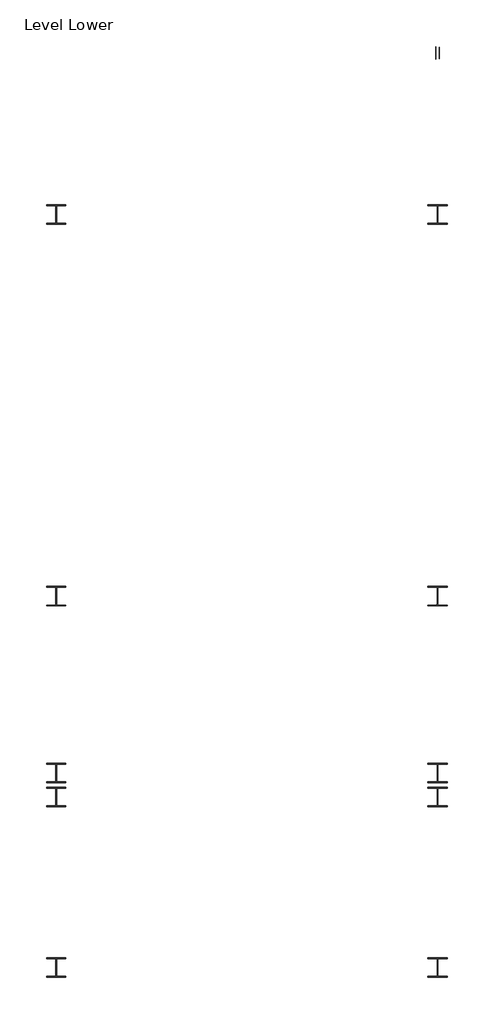
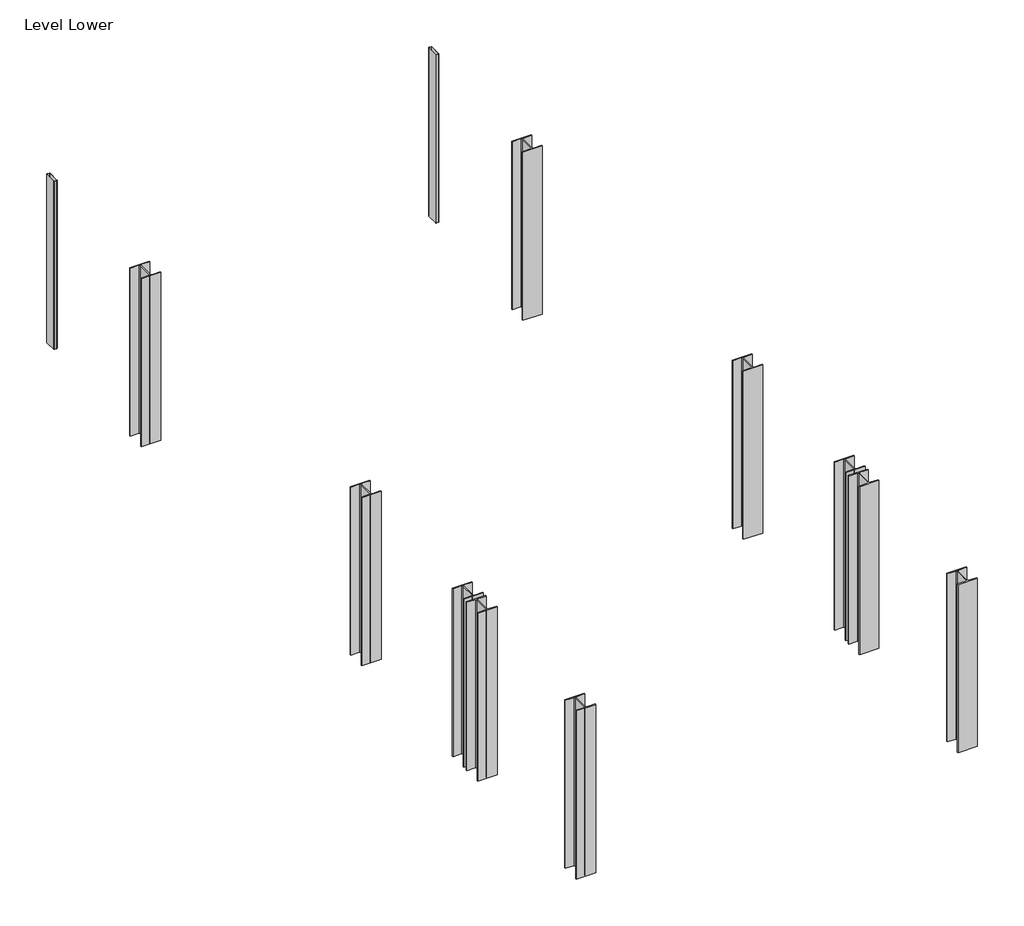
# One storey: 12 columns.
"""IFC4 building model written with IfcOpenShell, lengths in millimetres."""

import ifcopenshell
import ifcopenshell.guid

model = None  # the IFC model being written
_history = None  # IfcOwnerHistory: only IFC2X3 demands one
_inside = {}  # id of a spatial element -> (the spatial element, [elements in it])
_under = {}  # id of a project, library or spatial element -> (it, [spatial elements below it])
_declared = {}  # id of a project -> (the project, [libraries it declares])
_typed = {}  # id of a type object -> (the type object, [elements of that type])
_made_of = {}  # id of a material, layer set ... -> (it, [elements and type objects made of it])


def new_model(schema):
    """Start an empty IFC model of exactly this schema.

    Asked for "IFC4X3", IfcOpenShell would pick the latest addendum, in which some entities
    have other attributes; the version numbers below select the first issue.
    IFC2X3 requires an IfcOwnerHistory on every rooted entity: one is made here for all.
    """
    global model, _history
    if schema == "IFC4X3":
        model = ifcopenshell.file(schema_version=(4, 3, 0, 0))
    else:
        model = ifcopenshell.file(schema=schema)
    _inside.clear()
    _under.clear()
    _declared.clear()
    _typed.clear()
    _made_of.clear()
    _history = None
    if model.schema == "IFC2X3":
        org = make("IfcOrganization", Name="unknown")
        user = make(
            "IfcPersonAndOrganization",
            ThePerson=make("IfcPerson", FamilyName="unknown"),
            TheOrganization=org,
        )
        app = make(
            "IfcApplication",
            ApplicationDeveloper=org,
            Version="unknown",
            ApplicationFullName="unknown",
            ApplicationIdentifier="unknown",
        )
        _history = make(
            "IfcOwnerHistory",
            OwningUser=user,
            OwningApplication=app,
            ChangeAction="ADDED",
            CreationDate=0,
        )
    return model


def make(cls, **values):
    """One entity of the class cls with the attributes given. An attribute that is None is left unset."""
    return model.create_entity(
        cls, **{name: value for name, value in values.items() if value is not None}
    )


def rooted(cls, **values):
    """An entity with a GlobalId (a new one), such as an element, a storey or a relation."""
    return make(cls, GlobalId=ifcopenshell.guid.new(), OwnerHistory=_history, **values)


def si_unit(unit_type, name, prefix=None):
    """IfcSIUnit, for example si_unit("LENGTHUNIT", "METRE", prefix="MILLI")."""
    return make("IfcSIUnit", UnitType=unit_type, Prefix=prefix, Name=name)


def assignment(units):
    """IfcUnitAssignment: the units of a project."""
    return None if units is None else make("IfcUnitAssignment", Units=units)


def point(xyz):
    """IfcCartesianPoint."""
    return None if xyz is None else make("IfcCartesianPoint", Coordinates=xyz)


def direction(xyz):
    """IfcDirection."""
    return None if xyz is None else make("IfcDirection", DirectionRatios=xyz)


def frame(location, z_axis=None, x_axis=None):
    """IfcAxis2Placement3D, a coordinate frame: its origin and axes. An axis left out is left unset."""
    return make(
        "IfcAxis2Placement3D",
        Location=point(location),
        Axis=direction(z_axis),
        RefDirection=direction(x_axis),
    )


def frame_2d(location, x_axis=None):
    """IfcAxis2Placement2D, a coordinate frame in the plane: its origin and x axis."""
    return make(
        "IfcAxis2Placement2D", Location=point(location), RefDirection=direction(x_axis)
    )


def origin():
    """The frame at (0, 0, 0) with its axes left unset."""
    return frame((0.0, 0.0, 0.0))


def place(relative_to, where):
    """IfcLocalPlacement: puts the frame where relative to a parent placement (None: the world)."""
    return make(
        "IfcLocalPlacement", PlacementRelTo=relative_to, RelativePlacement=where
    )


def context(
    kind, dimensions, precision=None, world=None, true_north=None, identifier=None
):
    """IfcGeometricRepresentationContext, for example the 3D "Model" context."""
    return make(
        "IfcGeometricRepresentationContext",
        ContextIdentifier=identifier,
        ContextType=kind,
        CoordinateSpaceDimension=dimensions,
        Precision=precision,
        WorldCoordinateSystem=world,
        TrueNorth=true_north,
    )


def project(units=None, contexts=None):
    """IfcProject with its units and contexts."""
    return rooted(
        "IfcProject",
        Name="project",
        RepresentationContexts=contexts,
        UnitsInContext=assignment(units),
    )


def spatial(cls, under=None, at=None, **own):
    """A site, building, storey or space (cls), placed at a placement, below another one or the project."""
    s = rooted(cls, ObjectPlacement=at, **own)
    if under is not None:
        _under.setdefault(under.id(), (under, []))[1].append(s)
    return s


def polyline(points):
    """IfcPolyline through the points."""
    return make("IfcPolyline", Points=[point(p) for p in points])


def circle_curve(where, radius):
    """IfcCircle in the frame where."""
    return make("IfcCircle", Position=where, Radius=radius)


def trimmed(basis, trim1, trim2, sense, master):
    """IfcTrimmedCurve: the piece of a basis curve between two trims."""
    return make(
        "IfcTrimmedCurve",
        BasisCurve=basis,
        Trim1=trim1,
        Trim2=trim2,
        SenseAgreement=sense,
        MasterRepresentation=master,
    )


def segment(curve, same_sense, transition):
    """IfcCompositeCurveSegment."""
    return make(
        "IfcCompositeCurveSegment",
        Transition=transition,
        SameSense=same_sense,
        ParentCurve=curve,
    )


def composite_curve(segments, self_intersect=None):
    """IfcCompositeCurve: segments joined end to end."""
    return make("IfcCompositeCurve", Segments=segments, SelfIntersect=self_intersect)


def outline(outer, holes=None, kind="AREA"):
    """IfcArbitraryClosedProfileDef: a profile drawn as a closed curve; with holes, ...WithVoids."""
    if holes is None:
        return make("IfcArbitraryClosedProfileDef", ProfileType=kind, OuterCurve=outer)
    return make(
        "IfcArbitraryProfileDefWithVoids",
        ProfileType=kind,
        OuterCurve=outer,
        InnerCurves=holes,
    )


def extrude(swept, where, along, depth):
    """IfcExtrudedAreaSolid: the profile swept, set in the frame where, extruded along a direction by depth."""
    return make(
        "IfcExtrudedAreaSolid",
        SweptArea=swept,
        Position=where,
        ExtrudedDirection=direction(along),
        Depth=depth,
    )


def shape(context_of_items, identifier, shape_type, items):
    """IfcShapeRepresentation: the items that make up one representation, for example the "Body"."""
    return make(
        "IfcShapeRepresentation",
        ContextOfItems=context_of_items,
        RepresentationIdentifier=identifier,
        RepresentationType=shape_type,
        Items=items,
    )


def source(mapping_origin, context_of_items, identifier, shape_type, items):
    """IfcRepresentationMap: a shape defined once, which mapped items show again and again."""
    return make(
        "IfcRepresentationMap",
        MappingOrigin=mapping_origin,
        MappedRepresentation=shape(context_of_items, identifier, shape_type, items),
    )


def transform(
    local_origin,
    x_axis=None,
    y_axis=None,
    z_axis=None,
    scale=None,
    scale2=None,
    scale3=None,
    uniform=True,
):
    """IfcCartesianTransformationOperator3D, or its non-uniform kind. x_axis, y_axis, z_axis: its Axis1, 2, 3."""
    if uniform:
        return make(
            "IfcCartesianTransformationOperator3D",
            Axis1=direction(x_axis),
            Axis2=direction(y_axis),
            LocalOrigin=point(local_origin),
            Scale=scale,
            Axis3=direction(z_axis),
        )
    return make(
        "IfcCartesianTransformationOperator3DnonUniform",
        Axis1=direction(x_axis),
        Axis2=direction(y_axis),
        LocalOrigin=point(local_origin),
        Scale=scale,
        Axis3=direction(z_axis),
        Scale2=scale2,
        Scale3=scale3,
    )


def mapped(mapping_source, mapping_target):
    """IfcMappedItem: shows the shape of a source again, moved by a transform."""
    return make(
        "IfcMappedItem", MappingSource=mapping_source, MappingTarget=mapping_target
    )


def made_of(thing, what):
    """Note that an element or type object is made of a material, layer set ...; save() writes the relation."""
    if what is not None:
        _made_of.setdefault(what.id(), (what, []))[1].append(thing)
    return thing


def element(
    cls,
    number,
    at=None,
    inside=None,
    cuts=None,
    type_object=None,
    material=None,
    context=None,
    identifier="Body",
    shape_type=None,
    held_by="IfcProductDefinitionShape",
    body=None,
    shapes=None,
    **own,
):
    """One element of the class cls, such as IfcWall. Its Tag is "e" and its number.

    at: its placement. inside: the storey or other place that contains it. cuts: it is an
    opening in that element (IfcRelVoidsElement). A single representation is given by context,
    identifier, shape_type and body (its items); several are given by shapes. held_by: the class
    of the entity that holds the representations. save() writes the other relations.
    """
    e = rooted(cls, Tag="e%d" % number, ObjectPlacement=at, **own)
    if body is not None:
        shapes = [shape(context, identifier, shape_type, body)]
    if shapes is not None:
        e.Representation = make(held_by, Representations=shapes)
    if inside is not None:
        _inside.setdefault(inside.id(), (inside, []))[1].append(e)
    if cuts is not None:
        rooted(
            "IfcRelVoidsElement", RelatingBuildingElement=cuts, RelatedOpeningElement=e
        )
    if type_object is not None:
        _typed.setdefault(type_object.id(), (type_object, []))[1].append(e)
    return made_of(e, material)


def aggregate(whole, parts):
    """IfcRelAggregates: a whole, such as a stair, and the parts it consists of."""
    return rooted("IfcRelAggregates", RelatingObject=whole, RelatedObjects=parts)


def save(model, path):
    """Write the relations noted so far, then the file.

    IfcRelAggregates (storeys below a building ...), IfcRelContainedInSpatialStructure (elements
    in a storey), IfcRelDefinesByType, IfcRelAssociatesMaterial and IfcRelDeclares: one each for
    every whole, place, type object, material and project.
    """
    for whole, parts in _under.values():
        aggregate(whole, parts)
    for where, things in _inside.values():
        rooted(
            "IfcRelContainedInSpatialStructure",
            RelatedElements=things,
            RelatingStructure=where,
        )
    for kind, things in _typed.values():
        rooted("IfcRelDefinesByType", RelatedObjects=things, RelatingType=kind)
    for what, things in _made_of.values():
        rooted("IfcRelAssociatesMaterial", RelatedObjects=things, RelatingMaterial=what)
    for by, libraries in _declared.values():
        rooted("IfcRelDeclares", RelatingContext=by, RelatedDefinitions=libraries)
    model.write(path)


def hss_hollow_structural_section_column_hss8x2x3_16_e82f30fd(model_context):
    return source(origin(), model_context, "Body", "SweptSolid", [
        extrude(outline(composite_curve([segment(trimmed(circle_curve(frame_2d((16.5608, 92.7608)), 8.8392), [point((16.5608, 101.6))], [point((25.4, 92.7608))], False, "CARTESIAN"), True, "CONTINUOUS"), segment(polyline([(25.4, 92.7608), (25.4, -92.7608)]), True, "CONTINUOUS"), segment(trimmed(circle_curve(frame_2d((16.5608, -92.7608)), 8.8392), [point((25.4, -92.7608))], [point((16.5608, -101.6))], False, "CARTESIAN"), True, "CONTINUOUS"), segment(polyline([(16.5608, -101.6), (-16.5608, -101.6)]), True, "CONTINUOUS"), segment(trimmed(circle_curve(frame_2d((-16.5608, -92.7608)), 8.8392), [point((-16.5608, -101.6))], [point((-25.4, -92.7608))], False, "CARTESIAN"), True, "CONTINUOUS"), segment(polyline([(-25.4, -92.7608), (-25.4, 92.7608)]), True, "CONTINUOUS"), segment(trimmed(circle_curve(frame_2d((-16.5608, 92.7608)), 8.8392), [point((-25.4, 92.7608))], [point((-16.5608, 101.6))], False, "CARTESIAN"), True, "CONTINUOUS"), segment(polyline([(-16.5608, 101.6), (16.5608, 101.6)]), True, "CONTINUOUS")], self_intersect=False), holes=[composite_curve([segment(polyline([(16.5608, 97.1804), (-16.5608, 97.1804)]), True, "CONTINUOUS"), segment(trimmed(circle_curve(frame_2d((-16.5608, 92.7608)), 4.4196), [point((-16.5608, 97.1804))], [point((-20.9804, 92.7608))], True, "CARTESIAN"), True, "CONTINUOUS"), segment(polyline([(-20.9804, 92.7608), (-20.9804, -92.7608)]), True, "CONTINUOUS"), segment(trimmed(circle_curve(frame_2d((-16.5608, -92.7608)), 4.4196), [point((-20.9804, -92.7608))], [point((-16.5608, -97.1804))], True, "CARTESIAN"), True, "CONTINUOUS"), segment(polyline([(-16.5608, -97.1804), (16.5608, -97.1804)]), True, "CONTINUOUS"), segment(trimmed(circle_curve(frame_2d((16.5608, -92.7608)), 4.4196), [point((16.5608, -97.1804))], [point((20.9804, -92.7608))], True, "CARTESIAN"), True, "CONTINUOUS"), segment(polyline([(20.9804, -92.7608), (20.9804, 92.7608)]), True, "CONTINUOUS"), segment(trimmed(circle_curve(frame_2d((16.5608, 92.7608)), 4.4196), [point((20.9804, 92.7608))], [point((16.5608, 97.1804))], True, "CARTESIAN"), True, "CONTINUOUS")], self_intersect=False)]), frame((0.0, 0.0, -594.0), z_axis=(0.0, 0.0, 1.0), x_axis=(1.0, 0.0, 0.0)), (0.0, 0.0, 1.0), 2793.0),
    ])


def uc_universal_columns_column_uc305x305x97_6ea2ceb4(model_context):
    return source(origin(), model_context, "Body", "SweptSolid", [
        extrude(outline(composite_curve([segment(polyline([(152.65, 153.95), (152.65, 138.55), (20.15, 138.55)]), True, "CONTINUOUS"), segment(trimmed(circle_curve(frame_2d((20.15, 123.35)), 15.2), [point((20.15, 138.55))], [point((4.95, 123.35))], True, "CARTESIAN"), True, "CONTINUOUS"), segment(polyline([(4.95, 123.35), (4.95, -123.35)]), True, "CONTINUOUS"), segment(trimmed(circle_curve(frame_2d((20.15, -123.35)), 15.2), [point((4.95, -123.35))], [point((20.15, -138.55))], True, "CARTESIAN"), True, "CONTINUOUS"), segment(polyline([(20.15, -138.55), (152.65, -138.55), (152.65, -153.95), (-152.65, -153.95), (-152.65, -138.55), (-20.15, -138.55)]), True, "CONTINUOUS"), segment(trimmed(circle_curve(frame_2d((-20.15, -123.35)), 15.2), [point((-20.15, -138.55))], [point((-4.95, -123.35))], True, "CARTESIAN"), True, "CONTINUOUS"), segment(polyline([(-4.95, -123.35), (-4.95, 123.35)]), True, "CONTINUOUS"), segment(trimmed(circle_curve(frame_2d((-20.15, 123.35)), 15.2), [point((-4.95, 123.35))], [point((-20.15, 138.55))], True, "CARTESIAN"), True, "CONTINUOUS"), segment(polyline([(-20.15, 138.55), (-152.65, 138.55), (-152.65, 153.95), (152.65, 153.95)]), True, "CONTINUOUS")], self_intersect=False)), frame((0.0, 0.0, -594.0), z_axis=(0.0, 0.0, 1.0), x_axis=(1.0, 0.0, 0.0)), (0.0, 0.0, 1.0), 2793.0),
    ])


model = new_model("IFC4")

# Units and contexts
model_context = context("Model", 3, world=origin())
ifc_project = project(units=[si_unit("LENGTHUNIT", "METRE", prefix="MILLI")], contexts=[model_context])

# Site, building, storey
site = spatial("IfcSite", under=ifc_project)
building = spatial("IfcBuilding", under=site)
storey = spatial("IfcBuildingStorey", under=building, Name="Level Lower", Elevation=-550.0)

# Columns
placement = place(None, origin())
hss_hollow_structural_section_column_hss8x2x3_16_shape = hss_hollow_structural_section_column_hss8x2x3_16_e82f30fd(model_context)
element("IfcColumn", 1, ObjectType="HSS-Hollow Structural Section-Column : HSS8X2X3/16", at=placement, inside=storey, context=model_context, shape_type="MappedRepresentation", body=[
    mapped(hss_hollow_structural_section_column_hss8x2x3_16_shape, transform((7061.9315174, -3661.5939786, 0.0), x_axis=(1.0, 0.0, 0.0), y_axis=(0.0, 1.0, 0.0), z_axis=(0.0, 0.0, 1.0))),
])
element("IfcColumn", 2, ObjectType="HSS-Hollow Structural Section-Column : HSS8X2X3/16", at=placement, inside=storey, context=model_context, shape_type="MappedRepresentation", body=[
    mapped(hss_hollow_structural_section_column_hss8x2x3_16_shape, transform((13061.9315174, -3661.5939786, 0.0), x_axis=(1.0, 0.0, 0.0), y_axis=(0.0, 1.0, 0.0), z_axis=(0.0, 0.0, 1.0))),
])
uc_universal_columns_column_uc305x305x97_shape = uc_universal_columns_column_uc305x305x97_6ea2ceb4(model_context)
element("IfcColumn", 3, ObjectType="UC-Universal Columns-Column : UC305x305x97", at=placement, inside=storey, context=model_context, shape_type="MappedRepresentation", body=[
    mapped(uc_universal_columns_column_uc305x305x97_shape, transform((7061.9315174, -15361.5939786, 0.0), x_axis=(1.0, 0.0, 0.0), y_axis=(0.0, 1.0, 0.0), z_axis=(0.0, 0.0, 1.0))),
])
element("IfcColumn", 4, ObjectType="UC-Universal Columns-Column : UC305x305x97", at=placement, inside=storey, context=model_context, shape_type="MappedRepresentation", body=[
    mapped(uc_universal_columns_column_uc305x305x97_shape, transform((7061.9315174, -14981.5939786, 0.0), x_axis=(1.0, 0.0, 0.0), y_axis=(0.0, 1.0, 0.0), z_axis=(0.0, 0.0, 1.0))),
])
element("IfcColumn", 5, ObjectType="UC-Universal Columns-Column : UC305x305x97", at=placement, inside=storey, context=model_context, shape_type="MappedRepresentation", body=[
    mapped(uc_universal_columns_column_uc305x305x97_shape, transform((7061.9315174, -12201.5939786, 0.0), x_axis=(1.0, 0.0, 0.0), y_axis=(0.0, 1.0, 0.0), z_axis=(0.0, 0.0, 1.0))),
])
element("IfcColumn", 6, ObjectType="UC-Universal Columns-Column : UC305x305x97", at=placement, inside=storey, context=model_context, shape_type="MappedRepresentation", body=[
    mapped(uc_universal_columns_column_uc305x305x97_shape, transform((7061.9315174, -6201.5939786, 0.0), x_axis=(1.0, 0.0, 0.0), y_axis=(0.0, 1.0, 0.0), z_axis=(0.0, 0.0, 1.0))),
])
element("IfcColumn", 7, ObjectType="UC-Universal Columns-Column : UC305x305x97", at=placement, inside=storey, context=model_context, shape_type="MappedRepresentation", body=[
    mapped(uc_universal_columns_column_uc305x305x97_shape, transform((7061.9315174, -18041.5939786, 0.0), x_axis=(1.0, 0.0, 0.0), y_axis=(0.0, 1.0, 0.0), z_axis=(0.0, 0.0, 1.0))),
])
element("IfcColumn", 8, ObjectType="UC-Universal Columns-Column : UC305x305x97", at=placement, inside=storey, context=model_context, shape_type="MappedRepresentation", body=[
    mapped(uc_universal_columns_column_uc305x305x97_shape, transform((13061.9315174, -15361.5939786, 0.0), x_axis=(1.0, 0.0, 0.0), y_axis=(0.0, 1.0, 0.0), z_axis=(0.0, 0.0, 1.0))),
])
element("IfcColumn", 9, ObjectType="UC-Universal Columns-Column : UC305x305x97", at=placement, inside=storey, context=model_context, shape_type="MappedRepresentation", body=[
    mapped(uc_universal_columns_column_uc305x305x97_shape, transform((13061.9315174, -14981.5939786, 0.0), x_axis=(1.0, 0.0, 0.0), y_axis=(0.0, 1.0, 0.0), z_axis=(0.0, 0.0, 1.0))),
])
element("IfcColumn", 10, ObjectType="UC-Universal Columns-Column : UC305x305x97", at=placement, inside=storey, context=model_context, shape_type="MappedRepresentation", body=[
    mapped(uc_universal_columns_column_uc305x305x97_shape, transform((13061.9315174, -12201.5939786, 0.0), x_axis=(1.0, 0.0, 0.0), y_axis=(0.0, 1.0, 0.0), z_axis=(0.0, 0.0, 1.0))),
])
element("IfcColumn", 11, ObjectType="UC-Universal Columns-Column : UC305x305x97", at=placement, inside=storey, context=model_context, shape_type="MappedRepresentation", body=[
    mapped(uc_universal_columns_column_uc305x305x97_shape, transform((13061.9315174, -6201.5939786, 0.0), x_axis=(1.0, 0.0, 0.0), y_axis=(0.0, 1.0, 0.0), z_axis=(0.0, 0.0, 1.0))),
])
element("IfcColumn", 12, ObjectType="UC-Universal Columns-Column : UC305x305x97", at=placement, inside=storey, context=model_context, shape_type="MappedRepresentation", body=[
    mapped(uc_universal_columns_column_uc305x305x97_shape, transform((13061.9315174, -18041.5939786, 0.0), x_axis=(1.0, 0.0, 0.0), y_axis=(0.0, 1.0, 0.0), z_axis=(0.0, 0.0, 1.0))),
])

save(model, "model.ifc")

# Revit data of these elements
# Type "HSS-Hollow Structural Section-Column : HSS8X2X3/16"
#   Assembly Code = "B10"
#   Shape = "Rect."
#   Cost = 1
#   W = 12
#   Ht = 203.2 mm
#   b = 50.8 mm
#   kr = 8.839 mm
#   t = 4.42 mm
#   A = 0.00211612 m²
#   Structural Material [instance default] = Steel ASTM A500, Grade B, Rectangular and Square
# Type "UC-Universal Columns-Column : UC305x305x97"
#   Section Name Key = "UC305x305x97"
#   Cost = 5
#   Width = 30.53 cm
#   Web Thickness = 0.99 cm
#   Web Fillet = 1.52 cm
#   Warping Constant = 1560000.0 cm⁶
#   Torsional Moment of Inertia = 91.20 cm⁴
#   Section Area = 123.0 cm²
#   Plastic Modulus weak axis = 726.0 cm³
#   Plastic Modulus strong axis = 1592.0 cm³
#   Nominal Weight = 96.8996 kgf/m
#   Moment of Inertia weak axis = 7308.00 cm⁴
#   Moment of Inertia strong axis = 22249.00 cm⁴
#   Height = 30.79 cm
#   Flange Thickness = 1.54 cm
#   Elastic Modulus weak axis = 479.0 cm³
#   Elastic Modulus strong axis = 1445.0 cm³
#   Centroid Vertical = 15.395 cm
#   Centroid Horizontal = 15.265 cm
#   Bolt Spacing = 14.0 cm
#   Structural Material [instance default] = Metal - Steel 43-275
#   Type Comments = ""
#   Assembly Code = ""
# Elements 1, 2 (IfcColumn, "HSS-Hollow Structural Section-Column : HSS8X2X3/16")
#   Structural Material = Metal - Steel 43-275
#   Phase Created = New Construction
#   Materials on its faces: "Metal - Steel 43-275"
# Elements 3, 4, 5, 6, 7, 8, 9, 10, 11, 12 (IfcColumn, "UC-Universal Columns-Column : UC305x305x97")
#   Structural Material = Metal - Steel 43-275
#   Phase Created = New Construction
#   Materials on its faces: "Metal - Steel 43-275"
# Materials
#   "Steel ASTM A500, Grade B, Rectangular and Square": class "Metal", colour RGB 199 199 199, transparency 0, Description = "Carbon steel", Cost = 0
#   "Metal - Steel 43-275": class "Metal", colour RGB 247 247 247, transparency 0, Cost = 0
